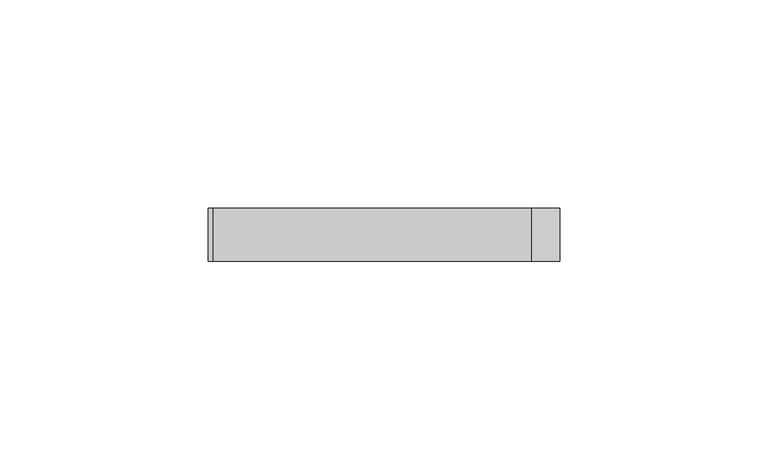
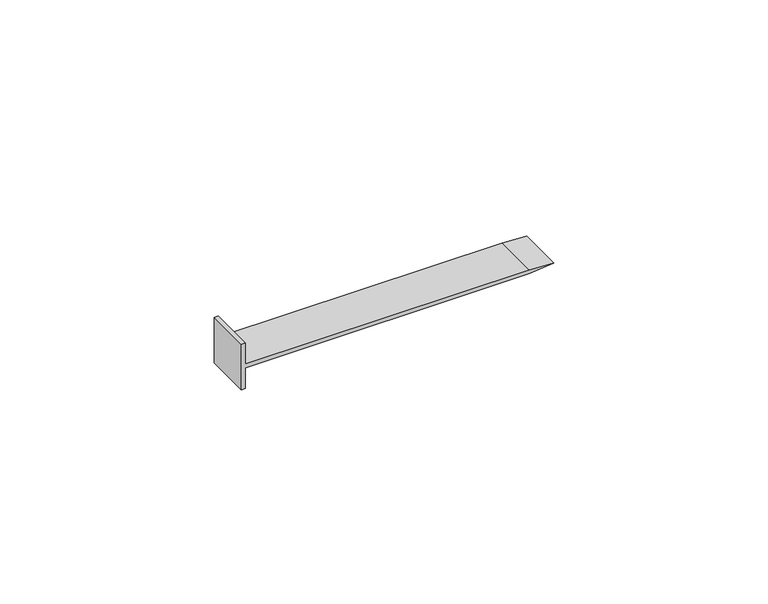
"""IFC4 building model written with IfcOpenShell, lengths in millimetres: proxy geometry, STAINLESS STEEL NAILS011 4116 : STAINLESS STEEL NAILS011 4116."""

from ifc_helpers import new_model, si_unit, frame, origin, place, context, project, spatial, polyline, outline, extrude, source, transform, mapped, element, save


def generic_models_70ec1e65(model_context):
    return source(origin(), model_context, "Body", "SweptSolid", [
        extrude(outline(polyline([(40201.6774651, -2804.8634295), (40201.6774651, -2803.7802308), (40207.6350577, -2803.7802308), (40207.6350577, -2727.2141564), (40208.3564507, -2720.5849902), (40208.7182563, -2727.2141564), (40208.7182563, -2803.7802308), (40214.675849, -2803.7802308), (40214.675849, -2804.8634295), (40201.6774651, -2804.8634295)])), frame((0.0, -1065.5906573, 0.0), z_axis=(0.0, 1.0, 0.0), x_axis=(0.0, 0.0, 1.0)), (0.0, 0.0, 1.0), 12.7),
    ])


if __name__ == "__main__":
    model = new_model("IFC4")
    model_context = context("Model", 3, world=origin())
    ifc_project = project(units=[si_unit("LENGTHUNIT", "METRE", prefix="MILLI")], contexts=[model_context])
    site = spatial("IfcSite", under=ifc_project)
    building = spatial("IfcBuilding", under=site)
    placement = place(None, origin())
    generic_models_shape = generic_models_70ec1e65(model_context)
    element("IfcBuildingElementProxy", 1, Name="STAINLESS STEEL NAILS011 4116 : STAINLESS STEEL NAILS011 4116", ObjectType="STAINLESS STEEL NAILS011 4116 : STAINLESS STEEL NAILS011 4116", at=placement, inside=building, context=model_context, shape_type="MappedRepresentation", body=[
        mapped(generic_models_shape, transform((0.0, 0.0, 0.0), x_axis=(1.0, 0.0, 0.0), y_axis=(0.0, 1.0, 0.0), z_axis=(0.0, 0.0, 1.0))),
    ])
    save(model, "model.ifc")

# Revit data of these elements
# Type "STAINLESS STEEL NAILS011 4116 : STAINLESS STEEL NAILS011 4116"
#   NameOverride = "STAINLESS STEEL NAILS011"
# Element 1 (IfcBuildingElementProxy, "STAINLESS STEEL NAILS011 4116 : STAINLESS STEEL NAILS011 4116")
#   Materials on its faces: "1 3/4\" STAINLESS STEEL RINGSHANK 5D COMMON NAILS @ 4\" (101.6MM) O.C. FIRESTONE PROVIDED MAX., 1/2\" STAGGERED"
# Materials
#   "1 3/4\" STAINLESS STEEL RINGSHANK 5D COMMON NAILS @ 4\" (101.6MM) O.C. FIRESTONE PROVIDED MAX., 1/2\" STAGGERED": class "Unassigned", colour RGB 255 255 255, transparency 0
